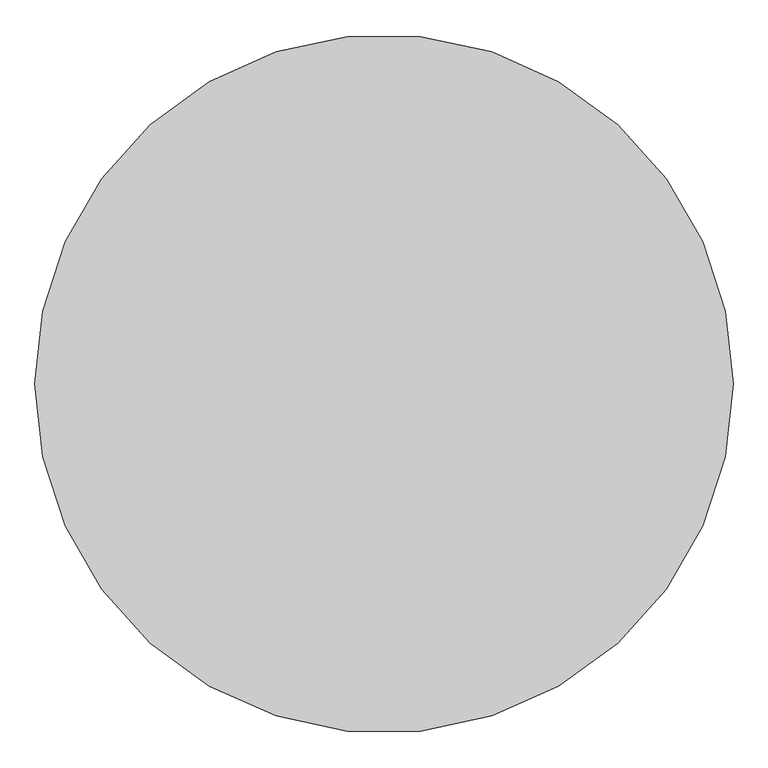
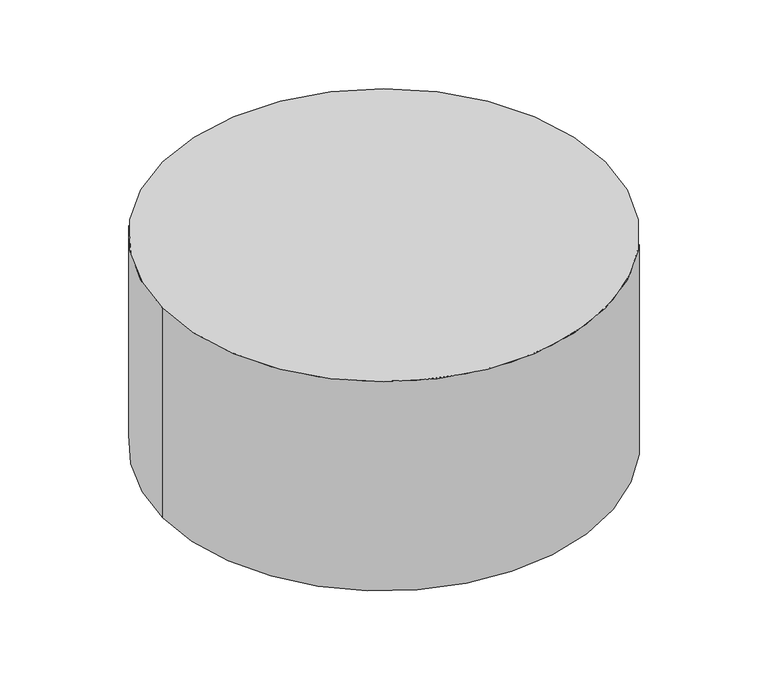
"""IFC4 building model written with IfcOpenShell, lengths in millimetres: proxy geometry, 일반 모델 3 : 일반 모델 3."""

from ifc_helpers import new_model, si_unit, point, frame, frame_2d, origin, place, context, project, spatial, circle_curve, trimmed, segment, composite_curve, outline, extrude, source, transform, mapped, element, save


def generic_models_b146cfb7(model_context):
    return source(origin(), model_context, "Body", "SweptSolid", [
        extrude(outline(composite_curve([segment(trimmed(circle_curve(frame_2d((586.4784316, 1589.1761456)), 1100.0), [point((-513.5215684, 1589.1761456))], [point((1686.4784316, 1589.1761456))], False, "CARTESIAN"), True, "CONTINUOUS"), segment(trimmed(circle_curve(frame_2d((586.4784316, 1589.1761456)), 1100.0), [point((1686.4784316, 1589.1761456))], [point((-513.5215684, 1589.1761456))], False, "CARTESIAN"), True, "CONTINUOUS")], self_intersect=False)), frame((0.0, 0.0, 250.0), z_axis=(0.0, 0.0, 1.0), x_axis=(1.0, 0.0, 0.0)), (0.0, 0.0, 1.0), 1100.0),
    ])


if __name__ == "__main__":
    model = new_model("IFC4")
    model_context = context("Model", 3, world=origin())
    ifc_project = project(units=[si_unit("LENGTHUNIT", "METRE", prefix="MILLI")], contexts=[model_context])
    site = spatial("IfcSite", under=ifc_project)
    building = spatial("IfcBuilding", under=site)
    placement = place(None, origin())
    generic_models_shape = generic_models_b146cfb7(model_context)
    element("IfcBuildingElementProxy", 1, Name="일반 모델 3 : 일반 모델 3", ObjectType="일반 모델 3 : 일반 모델 3", at=placement, inside=building, context=model_context, shape_type="MappedRepresentation", body=[
        mapped(generic_models_shape, transform((0.0, 0.0, 0.0), x_axis=(1.0, 0.0, 0.0), y_axis=(0.0, 1.0, 0.0), z_axis=(0.0, 0.0, 1.0))),
    ])
    save(model, "model.ifc")

# Revit data of these elements
# Type "일반 모델 3 : 일반 모델 3"
#   Type Mark = "StepLED.L.B.3"
# Element 1 (IfcBuildingElementProxy, "일반 모델 3 : 일반 모델 3")
#   Materials on its faces: "led_b"
# Materials
#   "led_b": class "일반", colour RGB 0 0 255, transparency 1, Cost = 0
